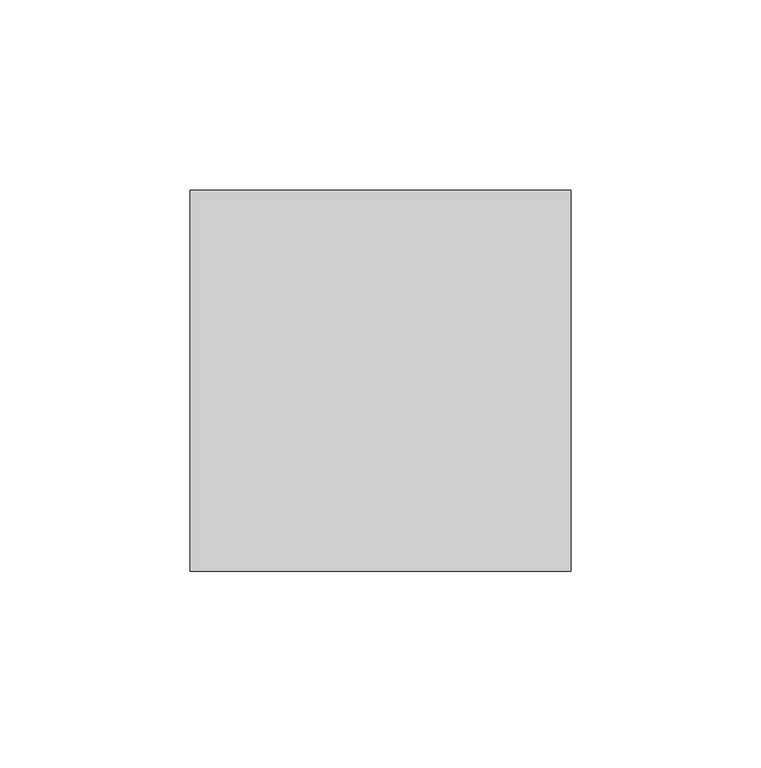
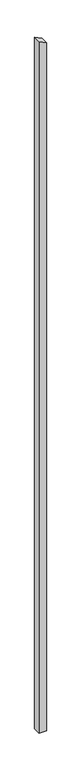
"""IFC4 building model written with IfcOpenShell, lengths in millimetres: column geometry, Holzstütze 159556 : Holzstütze 159556."""

from ifc_helpers import new_model, si_unit, frame, origin, place, context, project, spatial, polyline, outline, extrude, source, transform, mapped, element, save


def column_44b88cc2(model_context):
    return source(origin(), model_context, "Body", "SweptSolid", [
        extrude(outline(polyline([(-500.0, 168257.7593015), (-500.0, 168357.7593015), (9372.2929958, 168357.7593015), (9423.2455407, 168257.7593015), (-500.0, 168257.7593015)])), frame((0.0, 26981.9343946, 0.0), z_axis=(0.0, 1.0, 0.0), x_axis=(0.0, 0.0, 1.0)), (0.0, 0.0, 1.0), 100.0),
    ])


if __name__ == "__main__":
    model = new_model("IFC4")
    model_context = context("Model", 3, world=origin())
    ifc_project = project(units=[si_unit("LENGTHUNIT", "METRE", prefix="MILLI")], contexts=[model_context])
    site = spatial("IfcSite", under=ifc_project)
    building = spatial("IfcBuilding", under=site)
    placement = place(None, origin())
    column_shape = column_44b88cc2(model_context)
    element("IfcColumn", 1, ObjectType="Holzstütze 159556 : Holzstütze 159556", at=placement, inside=building, context=model_context, shape_type="MappedRepresentation", body=[
        mapped(column_shape, transform((0.0, 0.0, 0.0), x_axis=(1.0, 0.0, 0.0), y_axis=(0.0, 1.0, 0.0), z_axis=(0.0, 0.0, 1.0))),
    ])
    save(model, "model.ifc")

# Revit data of these elements
# Type "Holzstütze 159556 : Holzstütze 159556"
#   Abrechnungsart = "m"
#   Allright_Bauteil_ID = "0152St 0000143461"
#   Bezeichnung = "Holzstütze"
#   Codetext = "ST-HOLZ\\"
#   Gewerk = "Zimmer- und Holzbauarbeiten"
#   Material = "Holz"
#   Objektname = "Stütze"
#   NameOverride = "Holzstütze"
#   Reference = "Holzstütze"
#   Status = "NEW"
#   ThermalTransmittance = 0.0000 BTU/(h·ft²·°F)
#   Roll = 0.00°
#   Slope = 0.00°
#   2D Interaktion = yes
#   IsExternal = yes
#   LoadBearing = yes
# Element 1 (IfcColumn, "Holzstütze 159556 : Holzstütze 159556")
#   Materials on its faces: "holzschalung"
# Materials
#   "holzschalung": class "Unassigned", colour RGB 128 128 128, transparency 0
